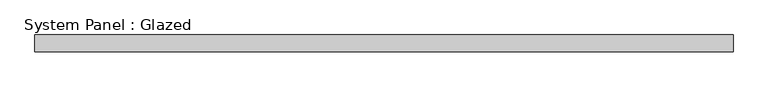
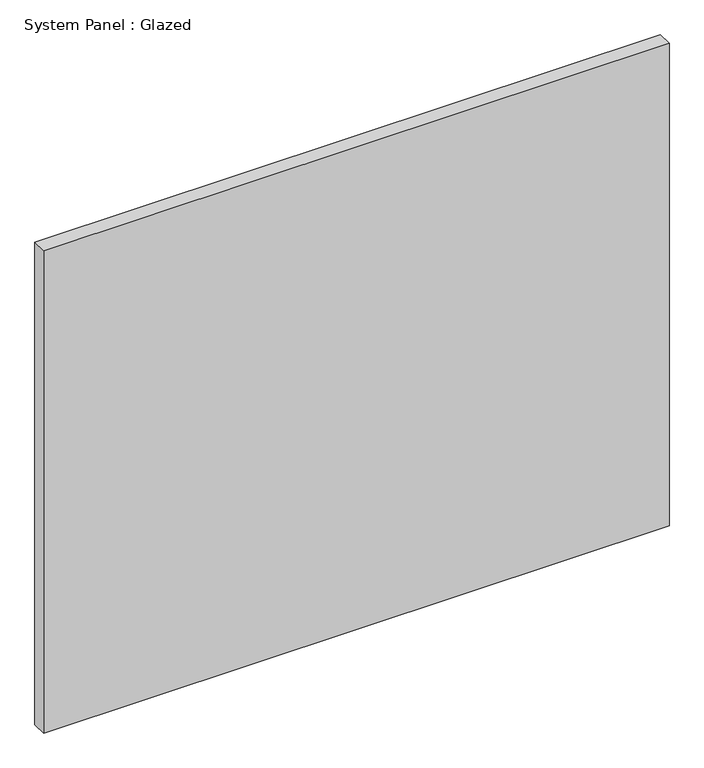
"""IFC4 building model written with IfcOpenShell, lengths in millimetres: plate geometry, System Panel : Glazed."""

from ifc_helpers import new_model, si_unit, origin, origin_with_axes, place, context, project, spatial, polyline, outline, extrude, source, transform, mapped, element, save


def system_panel_glazed_5b8ca2f9(model_context):
    return source(origin(), model_context, "Body", "SweptSolid", [
        extrude(outline(polyline([(533.4, 19.05), (-533.4, 19.05), (-533.4, 44.45), (533.4, 44.45), (533.4, 19.05)])), origin_with_axes(), (0.0, 0.0, 1.0), 869.95),
    ])


if __name__ == "__main__":
    model = new_model("IFC4")
    model_context = context("Model", 3, world=origin())
    ifc_project = project(units=[si_unit("LENGTHUNIT", "METRE", prefix="MILLI")], contexts=[model_context])
    site = spatial("IfcSite", under=ifc_project)
    building = spatial("IfcBuilding", under=site)
    placement = place(None, origin())
    system_panel_glazed_shape = system_panel_glazed_5b8ca2f9(model_context)
    element("IfcPlate", 1, ObjectType="System Panel : Glazed", at=placement, inside=building, context=model_context, shape_type="MappedRepresentation", body=[
        mapped(system_panel_glazed_shape, transform((0.0, 0.0, 0.0), x_axis=(1.0, 0.0, 0.0), y_axis=(0.0, 1.0, 0.0), z_axis=(0.0, 0.0, 1.0))),
    ])
    save(model, "model.ifc")

# Revit data of these elements
# Element 1 (IfcPlate, "System Panel : Glazed")
#   Materials on its faces: "Glass"
# Materials
#   "Glass": class "Glass", colour RGB 0 128 192, transparency 0.75
